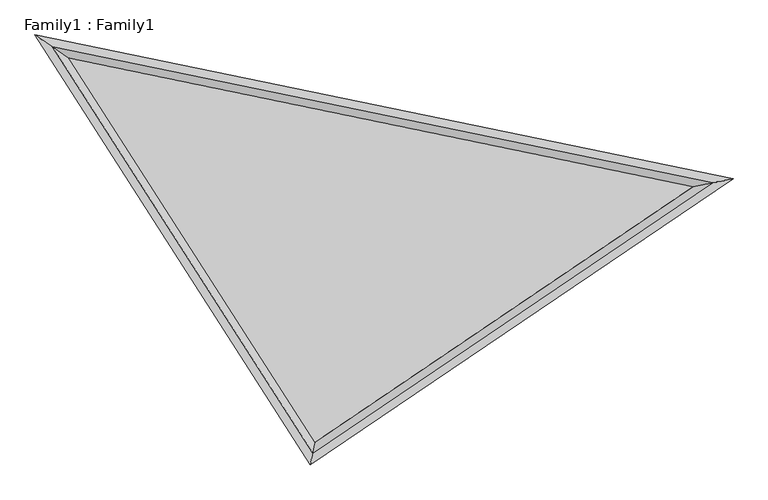
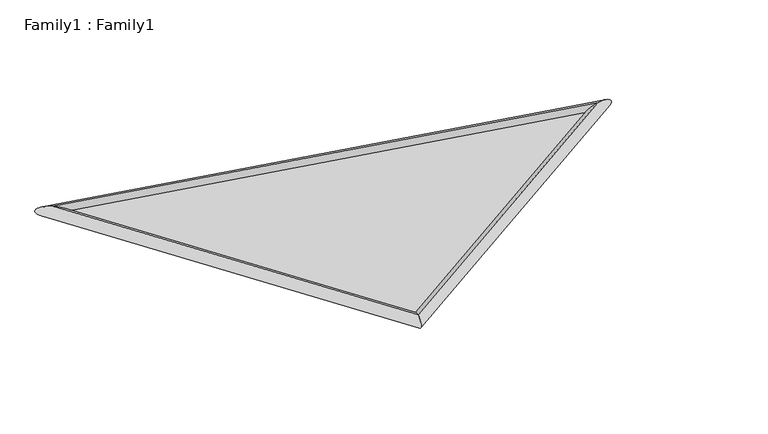
"""IFC4 building model written with IfcOpenShell, lengths in millimetres: proxy geometry, Family1 : Family1."""

from ifc_helpers import new_model, si_unit, frame, origin, origin_with_axes, place, context, project, spatial, polyline, ellipse_curve, outline, extrude, source, transform, mapped, element, save
from ifc_brep_helpers import cylinder_surface, advanced_brep


def family1_family1_2174ec98(model_context):
    return source(origin(), model_context, "Body", "SolidModel", [
        extrude(outline(polyline([(349.9363626, -2316.6838974), (-2857.7474921, 2688.1097571), (5274.7335806, 1012.5153452), (349.9363626, -2316.6838974)])), origin_with_axes(), (0.0, 0.0, 1.0), 34.1328789),
        advanced_brep(
        [(349.9363626, -2316.6838974, 100.0), (349.9363626, -2316.6838974, -100.0), (-2857.7474921, 2688.1097571, -100.0), (-2857.7474921, 2688.1097571, 100.0), (5274.7335806, 1012.5153452, -100.0), (5274.7335806, 1012.5153452, 100.0)],
        [
            (0, 1, ellipse_curve(frame((349.9363626, -2316.6838974, 0.0), z_axis=(-0.9794270591212653, 0.20179850311900122, 0.0), x_axis=(-0.20179850311900105, -0.9794270591212653, 0.0)), 143.1841912, 100.0)),
            (1, 2),
            (2, 3, ellipse_curve(frame((-2857.7474921, 2688.1097571, 0.0), z_axis=(-0.566301478842309, -0.8241981770551386, 0.0), x_axis=(0.8241981770551386, -0.5663014788423091, 0.0)), 257.5135809, 100.0)),
            (3, 0),
            (1, 0, ellipse_curve(frame((349.9363626, -2316.6838974, 0.0), z_axis=(-0.9794270591212653, 0.20179850311900122, 0.0), x_axis=(-0.20179850311900105, -0.9794270591212653, 0.0)), 143.1841912, 100.0)),
            (3, 2, ellipse_curve(frame((-2857.7474921, 2688.1097571, 0.0), z_axis=(-0.566301478842309, -0.8241981770551386, 0.0), x_axis=(0.8241981770551386, -0.5663014788423091, 0.0)), 257.5135809, 100.0)),
            (2, 4),
            (4, 5, ellipse_curve(frame((5274.7335806, 1012.5153452, 0.0), z_axis=(-0.19437844784920066, 0.9809266124495427, 0.0), x_axis=(-0.9809266124495428, -0.19437844784920053, 0.0)), 257.5135809, 100.0)),
            (5, 3),
            (5, 4, ellipse_curve(frame((5274.7335806, 1012.5153452, 0.0), z_axis=(-0.19437844784920066, 0.9809266124495427, 0.0), x_axis=(-0.9809266124495428, -0.19437844784920053, 0.0)), 257.5135809, 100.0)),
            (4, 1),
            (0, 5),
        ],
        [
            cylinder_surface(frame((349.9363626, -2316.6838974, 0.0), z_axis=(0.539604447116295, -0.8419186662928418, 0.0), x_axis=(-0.8419186662928418, -0.539604447116295, 0.0)), 100.0),
            cylinder_surface(frame((-2857.7474921, 2688.1097571, 0.0), z_axis=(-0.9794270591212653, 0.20179850311900127, 0.0), x_axis=(0.20179850311900127, 0.9794270591212653, 0.0)), 100.0),
            cylinder_surface(frame((5274.7335806, 1012.5153452, 0.0), z_axis=(0.8284614695111534, 0.5600460637620982, 0.0), x_axis=(0.5600460637620982, -0.8284614695111534, 0.0)), 100.0),
        ],
        [
            (0, [[1, 2, 3, 4]]),
            (0, [[5, -4, 6, -2]]),
            (1, [[-3, 7, 8, 9]]),
            (1, [[-6, -9, 10, -7]]),
            (2, [[-8, 11, -1, 12]]),
            (2, [[-10, -12, -5, -11]]),
        ],
    ),
    ])


if __name__ == "__main__":
    model = new_model("IFC4")
    model_context = context("Model", 3, world=origin())
    ifc_project = project(units=[si_unit("LENGTHUNIT", "METRE", prefix="MILLI")], contexts=[model_context])
    site = spatial("IfcSite", under=ifc_project)
    building = spatial("IfcBuilding", under=site)
    placement = place(None, origin())
    family1_family1_shape = family1_family1_2174ec98(model_context)
    element("IfcBuildingElementProxy", 1, Name="Family1 : Family1", ObjectType="Family1 : Family1", at=placement, inside=building, context=model_context, shape_type="MappedRepresentation", body=[
        mapped(family1_family1_shape, transform((0.0, 0.0, 0.0), x_axis=(1.0, 0.0, 0.0), y_axis=(0.0, 1.0, 0.0), z_axis=(0.0, 0.0, 1.0))),
    ])
    save(model, "model.ifc")

# Revit data of these elements
# Type "Family1 : Family1"
#   Default Elevation = 0
# Element 1 (IfcBuildingElementProxy, "Family1 : Family1")
#   Materials on its faces: "Glass"
# Materials
#   "Glass": class "Glass", colour RGB 0 128 192, transparency 0.9, Description = "Soda Lime Glass", Cost = 0
